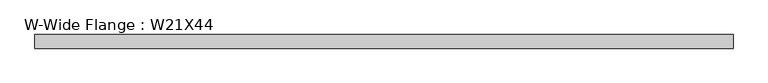
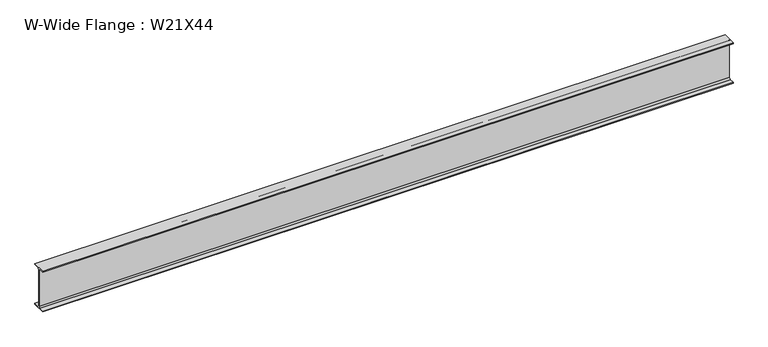
"""IFC4 building model written with IfcOpenShell, lengths in millimetres: beam geometry, W-Wide Flange : W21X44."""

from ifc_helpers import new_model, si_unit, point, frame, frame_2d, origin, place, context, project, spatial, polyline, circle_curve, trimmed, segment, composite_curve, outline, extrude, source, transform, mapped, element, save


def w_wide_flange_w21x44_feb090a0(model_context):
    return source(origin(), model_context, "Body", "SweptSolid", [
        extrude(outline(composite_curve([segment(polyline([(82.55, -251.46), (82.55, -262.89), (-82.55, -262.89), (-82.55, -251.46), (-21.59, -251.46)]), True, "CONTINUOUS"), segment(trimmed(circle_curve(frame_2d((-21.59, -234.315)), 17.145), [point((-21.59, -251.46))], [point((-4.445, -234.315))], True, "CARTESIAN"), True, "CONTINUOUS"), segment(polyline([(-4.445, -234.315), (-4.445, 234.315)]), True, "CONTINUOUS"), segment(trimmed(circle_curve(frame_2d((-21.59, 234.315)), 17.145), [point((-4.445, 234.315))], [point((-21.59, 251.46))], True, "CARTESIAN"), True, "CONTINUOUS"), segment(polyline([(-21.59, 251.46), (-82.55, 251.46), (-82.55, 262.89), (82.55, 262.89), (82.55, 251.46), (21.59, 251.46)]), True, "CONTINUOUS"), segment(trimmed(circle_curve(frame_2d((21.59, 234.315)), 17.145), [point((21.59, 251.46))], [point((4.445, 234.315))], True, "CARTESIAN"), True, "CONTINUOUS"), segment(polyline([(4.445, 234.315), (4.445, -234.315)]), True, "CONTINUOUS"), segment(trimmed(circle_curve(frame_2d((21.59, -234.315)), 17.145), [point((4.445, -234.315))], [point((21.59, -251.46))], True, "CARTESIAN"), True, "CONTINUOUS"), segment(polyline([(21.59, -251.46), (82.55, -251.46)]), True, "CONTINUOUS")], self_intersect=False)), frame((-4220.21, 0.0, 0.0), z_axis=(1.0, 0.0, 0.0), x_axis=(0.0, 1.0, 0.0)), (0.0, 0.0, 1.0), 8440.42),
    ])


if __name__ == "__main__":
    model = new_model("IFC4")
    model_context = context("Model", 3, world=origin())
    ifc_project = project(units=[si_unit("LENGTHUNIT", "METRE", prefix="MILLI")], contexts=[model_context])
    site = spatial("IfcSite", under=ifc_project)
    building = spatial("IfcBuilding", under=site)
    placement = place(None, origin())
    w_wide_flange_w21x44_shape = w_wide_flange_w21x44_feb090a0(model_context)
    element("IfcBeam", 1, ObjectType="W-Wide Flange : W21X44", at=placement, inside=building, context=model_context, shape_type="MappedRepresentation", body=[
        mapped(w_wide_flange_w21x44_shape, transform((0.0, 0.0, 0.0), x_axis=(1.0, 0.0, 0.0), y_axis=(0.0, 1.0, 0.0), z_axis=(0.0, 0.0, 1.0))),
    ])
    save(model, "model.ifc")

# Revit data of these elements
# Type "W-Wide Flange : W21X44"
#   Assembly Code = "B10"
#   W = 44
#   Start Extension Calculation [instance default] = 10' - 0"
#   Start Extension [instance default] = -0' - 0 1/2"
#   End Extension Calculation [instance default] = 10' - 0"
#   End Extension [instance default] = -0' - 0 1/2"
#   Length [instance default] = 5' - 0"
#   bf = 0' - 6 1/2"
#   d = 1' - 8.7"
#   k = 0' - 1 1/8"
#   k2 = 0' - 0.675"
#   tf = 0' - 0.45"
#   tw = 0' - 0.35"
#   A = 0.0902778 SF
#   Beam Material [instance default] = Metal - Steel - ASTM A992
# Element 1 (IfcBeam, "W-Wide Flange : W21X44")
#   Materials on its faces: "Metal - Steel - ASTM A992"
# Materials
#   "Metal - Steel - ASTM A992": class "Metal", colour RGB 128 0 0, transparency 0
